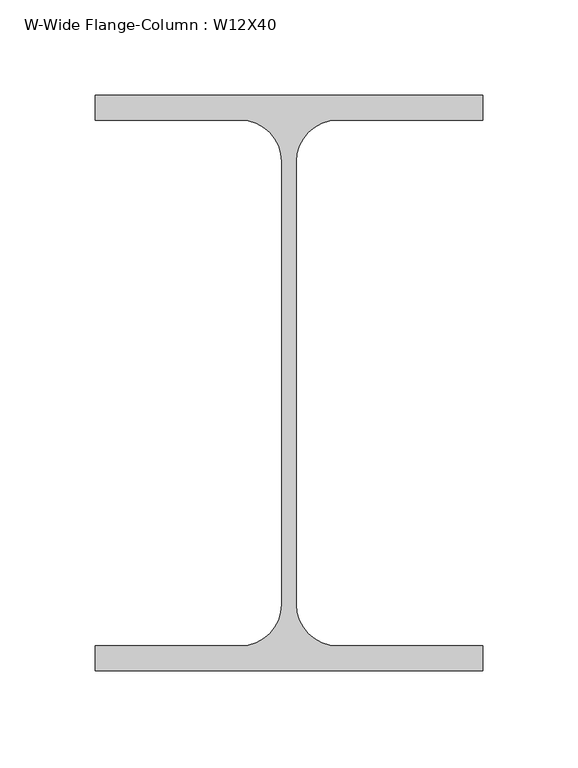
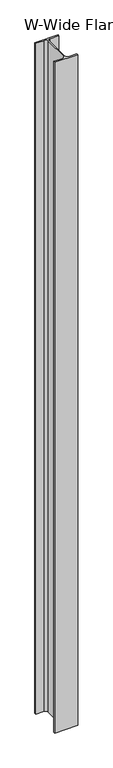
"""IFC4 building model written with IfcOpenShell, lengths in millimetres: column geometry, W-Wide Flange-Column : W12X40."""

from ifc_helpers import new_model, si_unit, point, frame, frame_2d, origin, place, context, project, spatial, polyline, circle_curve, trimmed, segment, composite_curve, outline, extrude, source, transform, mapped, element, save


def w_wide_flange_column_w12x40_573c2af4(model_context):
    return source(origin(), model_context, "Body", "SweptSolid", [
        extrude(outline(composite_curve([segment(polyline([(101.727, 151.13), (101.727, 138.049), (25.5905, 138.049)]), True, "CONTINUOUS"), segment(trimmed(circle_curve(frame_2d((25.5905, 116.205)), 21.844), [point((25.5905, 138.049))], [point((3.7465, 116.205))], True, "CARTESIAN"), True, "CONTINUOUS"), segment(polyline([(3.7465, 116.205), (3.7465, -116.205)]), True, "CONTINUOUS"), segment(trimmed(circle_curve(frame_2d((25.5905, -116.205)), 21.844), [point((3.7465, -116.205))], [point((25.5905, -138.049))], True, "CARTESIAN"), True, "CONTINUOUS"), segment(polyline([(25.5905, -138.049), (101.727, -138.049), (101.727, -151.13), (-101.727, -151.13), (-101.727, -138.049), (-25.5905, -138.049)]), True, "CONTINUOUS"), segment(trimmed(circle_curve(frame_2d((-25.5905, -116.205)), 21.844), [point((-25.5905, -138.049))], [point((-3.7465, -116.205))], True, "CARTESIAN"), True, "CONTINUOUS"), segment(polyline([(-3.7465, -116.205), (-3.7465, 116.205)]), True, "CONTINUOUS"), segment(trimmed(circle_curve(frame_2d((-25.5905, 116.205)), 21.844), [point((-3.7465, 116.205))], [point((-25.5905, 138.049))], True, "CARTESIAN"), True, "CONTINUOUS"), segment(polyline([(-25.5905, 138.049), (-101.727, 138.049), (-101.727, 151.13), (101.727, 151.13)]), True, "CONTINUOUS")], self_intersect=False)), frame((0.0, 0.0, 23317.2), z_axis=(0.0, 0.0, 1.0), x_axis=(1.0, 0.0, 0.0)), (0.0, 0.0, 1.0), 6248.4),
    ])


if __name__ == "__main__":
    model = new_model("IFC4")
    model_context = context("Model", 3, world=origin())
    ifc_project = project(units=[si_unit("LENGTHUNIT", "METRE", prefix="MILLI")], contexts=[model_context])
    site = spatial("IfcSite", under=ifc_project)
    building = spatial("IfcBuilding", under=site)
    placement = place(None, origin())
    w_wide_flange_column_w12x40_shape = w_wide_flange_column_w12x40_573c2af4(model_context)
    element("IfcColumn", 1, ObjectType="W-Wide Flange-Column : W12X40", at=placement, inside=building, context=model_context, shape_type="MappedRepresentation", body=[
        mapped(w_wide_flange_column_w12x40_shape, transform((0.0, 0.0, 0.0), x_axis=(1.0, 0.0, 0.0), y_axis=(0.0, 1.0, 0.0), z_axis=(0.0, 0.0, 1.0))),
    ])
    save(model, "model.ifc")

# Revit data of these elements
# Type "W-Wide Flange-Column : W12X40"
#   Assembly Code = "B10"
#   W = 40
#   bf = 0' - 8.01"
#   d = 0' - 11.9"
#   k = 0' - 1 3/8"
#   kr = 0' - 0.86"
#   tf = 0' - 0.515"
#   tw = 0' - 0.295"
#   A = 0.08125 SF
#   Structural Material [instance default] = Steel ASTM A992
# Element 1 (IfcColumn, "W-Wide Flange-Column : W12X40")
#   Materials on its faces: "Steel ASTM A992"
# Materials
#   "Steel ASTM A992": class "Metal", colour RGB 199 199 199, transparency 0, Description = "Structural steel 50ksi", Cost = 0
